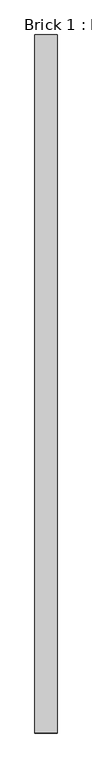
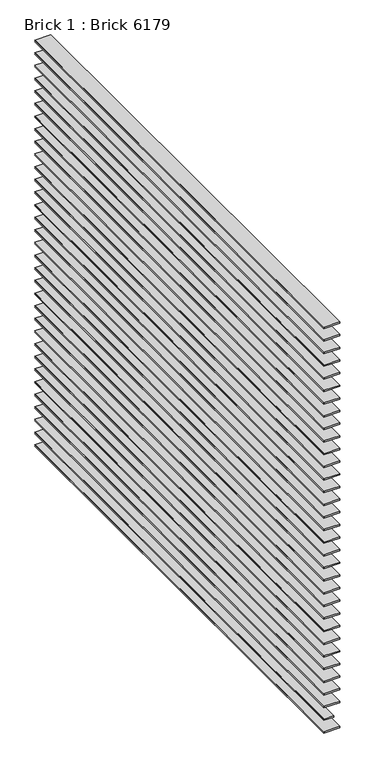
"""IFC4 building model written with IfcOpenShell, lengths in millimetres: proxy geometry, Brick 1 : Brick 6179."""

import ifcopenshell
import ifcopenshell.guid

model = None  # the IFC model being written
_history = None  # IfcOwnerHistory: only IFC2X3 demands one
_inside = {}  # id of a spatial element -> (the spatial element, [elements in it])
_under = {}  # id of a project, library or spatial element -> (it, [spatial elements below it])
_declared = {}  # id of a project -> (the project, [libraries it declares])
_typed = {}  # id of a type object -> (the type object, [elements of that type])
_made_of = {}  # id of a material, layer set ... -> (it, [elements and type objects made of it])


def new_model(schema):
    """Start an empty IFC model of exactly this schema.

    Asked for "IFC4X3", IfcOpenShell would pick the latest addendum, in which some entities
    have other attributes; the version numbers below select the first issue.
    IFC2X3 requires an IfcOwnerHistory on every rooted entity: one is made here for all.
    """
    global model, _history
    if schema == "IFC4X3":
        model = ifcopenshell.file(schema_version=(4, 3, 0, 0))
    else:
        model = ifcopenshell.file(schema=schema)
    _inside.clear()
    _under.clear()
    _declared.clear()
    _typed.clear()
    _made_of.clear()
    _history = None
    if model.schema == "IFC2X3":
        org = make("IfcOrganization", Name="unknown")
        user = make(
            "IfcPersonAndOrganization",
            ThePerson=make("IfcPerson", FamilyName="unknown"),
            TheOrganization=org,
        )
        app = make(
            "IfcApplication",
            ApplicationDeveloper=org,
            Version="unknown",
            ApplicationFullName="unknown",
            ApplicationIdentifier="unknown",
        )
        _history = make(
            "IfcOwnerHistory",
            OwningUser=user,
            OwningApplication=app,
            ChangeAction="ADDED",
            CreationDate=0,
        )
    return model


def make(cls, **values):
    """One entity of the class cls with the attributes given. An attribute that is None is left unset."""
    return model.create_entity(
        cls, **{name: value for name, value in values.items() if value is not None}
    )


def rooted(cls, **values):
    """An entity with a GlobalId (a new one), such as an element, a storey or a relation."""
    return make(cls, GlobalId=ifcopenshell.guid.new(), OwnerHistory=_history, **values)


def si_unit(unit_type, name, prefix=None):
    """IfcSIUnit, for example si_unit("LENGTHUNIT", "METRE", prefix="MILLI")."""
    return make("IfcSIUnit", UnitType=unit_type, Prefix=prefix, Name=name)


def assignment(units):
    """IfcUnitAssignment: the units of a project."""
    return None if units is None else make("IfcUnitAssignment", Units=units)


def point(xyz):
    """IfcCartesianPoint."""
    return None if xyz is None else make("IfcCartesianPoint", Coordinates=xyz)


def direction(xyz):
    """IfcDirection."""
    return None if xyz is None else make("IfcDirection", DirectionRatios=xyz)


def frame(location, z_axis=None, x_axis=None):
    """IfcAxis2Placement3D, a coordinate frame: its origin and axes. An axis left out is left unset."""
    return make(
        "IfcAxis2Placement3D",
        Location=point(location),
        Axis=direction(z_axis),
        RefDirection=direction(x_axis),
    )


def frame_2d(location, x_axis=None):
    """IfcAxis2Placement2D, a coordinate frame in the plane: its origin and x axis."""
    return make(
        "IfcAxis2Placement2D", Location=point(location), RefDirection=direction(x_axis)
    )


def origin():
    """The frame at (0, 0, 0) with its axes left unset."""
    return frame((0.0, 0.0, 0.0))


def place(relative_to, where):
    """IfcLocalPlacement: puts the frame where relative to a parent placement (None: the world)."""
    return make(
        "IfcLocalPlacement", PlacementRelTo=relative_to, RelativePlacement=where
    )


def context(
    kind, dimensions, precision=None, world=None, true_north=None, identifier=None
):
    """IfcGeometricRepresentationContext, for example the 3D "Model" context."""
    return make(
        "IfcGeometricRepresentationContext",
        ContextIdentifier=identifier,
        ContextType=kind,
        CoordinateSpaceDimension=dimensions,
        Precision=precision,
        WorldCoordinateSystem=world,
        TrueNorth=true_north,
    )


def project(units=None, contexts=None):
    """IfcProject with its units and contexts."""
    return rooted(
        "IfcProject",
        Name="project",
        RepresentationContexts=contexts,
        UnitsInContext=assignment(units),
    )


def spatial(cls, under=None, at=None, **own):
    """A site, building, storey or space (cls), placed at a placement, below another one or the project."""
    s = rooted(cls, ObjectPlacement=at, **own)
    if under is not None:
        _under.setdefault(under.id(), (under, []))[1].append(s)
    return s


def polyline(points):
    """IfcPolyline through the points."""
    return make("IfcPolyline", Points=[point(p) for p in points])


def circle_curve(where, radius):
    """IfcCircle in the frame where."""
    return make("IfcCircle", Position=where, Radius=radius)


def trimmed(basis, trim1, trim2, sense, master):
    """IfcTrimmedCurve: the piece of a basis curve between two trims."""
    return make(
        "IfcTrimmedCurve",
        BasisCurve=basis,
        Trim1=trim1,
        Trim2=trim2,
        SenseAgreement=sense,
        MasterRepresentation=master,
    )


def segment(curve, same_sense, transition):
    """IfcCompositeCurveSegment."""
    return make(
        "IfcCompositeCurveSegment",
        Transition=transition,
        SameSense=same_sense,
        ParentCurve=curve,
    )


def composite_curve(segments, self_intersect=None):
    """IfcCompositeCurve: segments joined end to end."""
    return make("IfcCompositeCurve", Segments=segments, SelfIntersect=self_intersect)


def outline(outer, holes=None, kind="AREA"):
    """IfcArbitraryClosedProfileDef: a profile drawn as a closed curve; with holes, ...WithVoids."""
    if holes is None:
        return make("IfcArbitraryClosedProfileDef", ProfileType=kind, OuterCurve=outer)
    return make(
        "IfcArbitraryProfileDefWithVoids",
        ProfileType=kind,
        OuterCurve=outer,
        InnerCurves=holes,
    )


def extrude(swept, where, along, depth):
    """IfcExtrudedAreaSolid: the profile swept, set in the frame where, extruded along a direction by depth."""
    return make(
        "IfcExtrudedAreaSolid",
        SweptArea=swept,
        Position=where,
        ExtrudedDirection=direction(along),
        Depth=depth,
    )


def shape(context_of_items, identifier, shape_type, items):
    """IfcShapeRepresentation: the items that make up one representation, for example the "Body"."""
    return make(
        "IfcShapeRepresentation",
        ContextOfItems=context_of_items,
        RepresentationIdentifier=identifier,
        RepresentationType=shape_type,
        Items=items,
    )


def source(mapping_origin, context_of_items, identifier, shape_type, items):
    """IfcRepresentationMap: a shape defined once, which mapped items show again and again."""
    return make(
        "IfcRepresentationMap",
        MappingOrigin=mapping_origin,
        MappedRepresentation=shape(context_of_items, identifier, shape_type, items),
    )


def transform(
    local_origin,
    x_axis=None,
    y_axis=None,
    z_axis=None,
    scale=None,
    scale2=None,
    scale3=None,
    uniform=True,
):
    """IfcCartesianTransformationOperator3D, or its non-uniform kind. x_axis, y_axis, z_axis: its Axis1, 2, 3."""
    if uniform:
        return make(
            "IfcCartesianTransformationOperator3D",
            Axis1=direction(x_axis),
            Axis2=direction(y_axis),
            LocalOrigin=point(local_origin),
            Scale=scale,
            Axis3=direction(z_axis),
        )
    return make(
        "IfcCartesianTransformationOperator3DnonUniform",
        Axis1=direction(x_axis),
        Axis2=direction(y_axis),
        LocalOrigin=point(local_origin),
        Scale=scale,
        Axis3=direction(z_axis),
        Scale2=scale2,
        Scale3=scale3,
    )


def mapped(mapping_source, mapping_target):
    """IfcMappedItem: shows the shape of a source again, moved by a transform."""
    return make(
        "IfcMappedItem", MappingSource=mapping_source, MappingTarget=mapping_target
    )


def made_of(thing, what):
    """Note that an element or type object is made of a material, layer set ...; save() writes the relation."""
    if what is not None:
        _made_of.setdefault(what.id(), (what, []))[1].append(thing)
    return thing


def element(
    cls,
    number,
    at=None,
    inside=None,
    cuts=None,
    type_object=None,
    material=None,
    context=None,
    identifier="Body",
    shape_type=None,
    held_by="IfcProductDefinitionShape",
    body=None,
    shapes=None,
    **own,
):
    """One element of the class cls, such as IfcWall. Its Tag is "e" and its number.

    at: its placement. inside: the storey or other place that contains it. cuts: it is an
    opening in that element (IfcRelVoidsElement). A single representation is given by context,
    identifier, shape_type and body (its items); several are given by shapes. held_by: the class
    of the entity that holds the representations. save() writes the other relations.
    """
    e = rooted(cls, Tag="e%d" % number, ObjectPlacement=at, **own)
    if body is not None:
        shapes = [shape(context, identifier, shape_type, body)]
    if shapes is not None:
        e.Representation = make(held_by, Representations=shapes)
    if inside is not None:
        _inside.setdefault(inside.id(), (inside, []))[1].append(e)
    if cuts is not None:
        rooted(
            "IfcRelVoidsElement", RelatingBuildingElement=cuts, RelatedOpeningElement=e
        )
    if type_object is not None:
        _typed.setdefault(type_object.id(), (type_object, []))[1].append(e)
    return made_of(e, material)


def aggregate(whole, parts):
    """IfcRelAggregates: a whole, such as a stair, and the parts it consists of."""
    return rooted("IfcRelAggregates", RelatingObject=whole, RelatedObjects=parts)


def save(model, path):
    """Write the relations noted so far, then the file.

    IfcRelAggregates (storeys below a building ...), IfcRelContainedInSpatialStructure (elements
    in a storey), IfcRelDefinesByType, IfcRelAssociatesMaterial and IfcRelDeclares: one each for
    every whole, place, type object, material and project.
    """
    for whole, parts in _under.values():
        aggregate(whole, parts)
    for where, things in _inside.values():
        rooted(
            "IfcRelContainedInSpatialStructure",
            RelatedElements=things,
            RelatingStructure=where,
        )
    for kind, things in _typed.values():
        rooted("IfcRelDefinesByType", RelatedObjects=things, RelatingType=kind)
    for what, things in _made_of.values():
        rooted("IfcRelAssociatesMaterial", RelatedObjects=things, RelatingMaterial=what)
    for by, libraries in _declared.values():
        rooted("IfcRelDeclares", RelatingContext=by, RelatedDefinitions=libraries)
    model.write(path)


def brick_1_brick_6179_25ec3522(model_context):
    return source(origin(), model_context, "Body", "SweptSolid", [
        extrude(outline(composite_curve([segment(polyline([(37320.25, 10083.0612048), (37326.2029111, 10083.0612048), (37326.2029111, 10019.5612048)]), True, "CONTINUOUS"), segment(trimmed(circle_curve(frame_2d((37323.2264555, 10016.8521801)), 4.0246867), [point((37326.2029111, 10019.5612048))], [point((37320.25, 10019.5612048))], True, "CARTESIAN"), True, "CONTINUOUS"), segment(polyline([(37320.25, 10019.5612048), (37320.25, 10083.0612048)]), True, "CONTINUOUS")], self_intersect=False)), frame((0.0, 2217.3609988, 0.0), z_axis=(0.0, 1.0, 0.0), x_axis=(0.0, 0.0, 1.0)), (0.0, 0.0, 1.0), 2000.0),
        extrude(outline(composite_curve([segment(polyline([(37373.6875, 10059.8947267), (37379.6404111, 10059.8947267), (37379.6404111, 10019.5612048)]), True, "CONTINUOUS"), segment(trimmed(circle_curve(frame_2d((37376.6639555, 10016.8521801)), 4.0246867), [point((37379.6404111, 10019.5612048))], [point((37373.6875, 10019.5612048))], True, "CARTESIAN"), True, "CONTINUOUS"), segment(polyline([(37373.6875, 10019.5612048), (37373.6875, 10059.8947267)]), True, "CONTINUOUS")], self_intersect=False)), frame((0.0, 2217.3609988, 0.0), z_axis=(0.0, 1.0, 0.0), x_axis=(0.0, 0.0, 1.0)), (0.0, 0.0, 1.0), 2000.0),
        extrude(outline(composite_curve([segment(polyline([(37427.125, 10083.0612048), (37433.0779111, 10083.0612048), (37433.0779111, 10019.5612048)]), True, "CONTINUOUS"), segment(trimmed(circle_curve(frame_2d((37430.1014555, 10016.8521801)), 4.0246867), [point((37433.0779111, 10019.5612048))], [point((37427.125, 10019.5612048))], True, "CARTESIAN"), True, "CONTINUOUS"), segment(polyline([(37427.125, 10019.5612048), (37427.125, 10083.0612048)]), True, "CONTINUOUS")], self_intersect=False)), frame((0.0, 2217.3609988, 0.0), z_axis=(0.0, 1.0, 0.0), x_axis=(0.0, 0.0, 1.0)), (0.0, 0.0, 1.0), 2000.0),
        extrude(outline(composite_curve([segment(polyline([(37480.5625, 10083.0612048), (37486.5154111, 10083.0612048), (37486.5154111, 10019.5612048)]), True, "CONTINUOUS"), segment(trimmed(circle_curve(frame_2d((37483.5389555, 10016.8521801)), 4.0246867), [point((37486.5154111, 10019.5612048))], [point((37480.5625, 10019.5612048))], True, "CARTESIAN"), True, "CONTINUOUS"), segment(polyline([(37480.5625, 10019.5612048), (37480.5625, 10083.0612048)]), True, "CONTINUOUS")], self_intersect=False)), frame((0.0, 2217.3609988, 0.0), z_axis=(0.0, 1.0, 0.0), x_axis=(0.0, 0.0, 1.0)), (0.0, 0.0, 1.0), 2000.0),
        extrude(outline(composite_curve([segment(polyline([(37534.0, 10083.0612048), (37539.9529111, 10083.0612048), (37539.9529111, 10019.5612048)]), True, "CONTINUOUS"), segment(trimmed(circle_curve(frame_2d((37536.9764555, 10016.8521801)), 4.0246867), [point((37539.9529111, 10019.5612048))], [point((37534.0, 10019.5612048))], True, "CARTESIAN"), True, "CONTINUOUS"), segment(polyline([(37534.0, 10019.5612048), (37534.0, 10083.0612048)]), True, "CONTINUOUS")], self_intersect=False)), frame((0.0, 2217.3609988, 0.0), z_axis=(0.0, 1.0, 0.0), x_axis=(0.0, 0.0, 1.0)), (0.0, 0.0, 1.0), 2000.0),
        extrude(outline(composite_curve([segment(polyline([(37587.4375, 10083.0612048), (37593.3904111, 10083.0612048), (37593.3904111, 10019.5612048)]), True, "CONTINUOUS"), segment(trimmed(circle_curve(frame_2d((37590.4139555, 10016.8521801)), 4.0246867), [point((37593.3904111, 10019.5612048))], [point((37587.4375, 10019.5612048))], True, "CARTESIAN"), True, "CONTINUOUS"), segment(polyline([(37587.4375, 10019.5612048), (37587.4375, 10083.0612048)]), True, "CONTINUOUS")], self_intersect=False)), frame((0.0, 2217.3609988, 0.0), z_axis=(0.0, 1.0, 0.0), x_axis=(0.0, 0.0, 1.0)), (0.0, 0.0, 1.0), 2000.0),
        extrude(outline(composite_curve([segment(polyline([(37640.875, 10083.0612048), (37646.8279111, 10083.0612048), (37646.8279111, 10019.5612048)]), True, "CONTINUOUS"), segment(trimmed(circle_curve(frame_2d((37643.8514555, 10016.8521801)), 4.0246867), [point((37646.8279111, 10019.5612048))], [point((37640.875, 10019.5612048))], True, "CARTESIAN"), True, "CONTINUOUS"), segment(polyline([(37640.875, 10019.5612048), (37640.875, 10083.0612048)]), True, "CONTINUOUS")], self_intersect=False)), frame((0.0, 2217.3609988, 0.0), z_axis=(0.0, 1.0, 0.0), x_axis=(0.0, 0.0, 1.0)), (0.0, 0.0, 1.0), 2000.0),
        extrude(outline(composite_curve([segment(polyline([(37694.3125, 10083.0612048), (37700.2654111, 10083.0612048), (37700.2654111, 10019.5612048)]), True, "CONTINUOUS"), segment(trimmed(circle_curve(frame_2d((37697.2889555, 10016.8521801)), 4.0246867), [point((37700.2654111, 10019.5612048))], [point((37694.3125, 10019.5612048))], True, "CARTESIAN"), True, "CONTINUOUS"), segment(polyline([(37694.3125, 10019.5612048), (37694.3125, 10083.0612048)]), True, "CONTINUOUS")], self_intersect=False)), frame((0.0, 2217.3609988, 0.0), z_axis=(0.0, 1.0, 0.0), x_axis=(0.0, 0.0, 1.0)), (0.0, 0.0, 1.0), 2000.0),
        extrude(outline(composite_curve([segment(polyline([(37747.75, 10083.0612048), (37753.7029111, 10083.0612048), (37753.7029111, 10019.5612048)]), True, "CONTINUOUS"), segment(trimmed(circle_curve(frame_2d((37750.7264555, 10016.8521801)), 4.0246867), [point((37753.7029111, 10019.5612048))], [point((37747.75, 10019.5612048))], True, "CARTESIAN"), True, "CONTINUOUS"), segment(polyline([(37747.75, 10019.5612048), (37747.75, 10083.0612048)]), True, "CONTINUOUS")], self_intersect=False)), frame((0.0, 2217.3609988, 0.0), z_axis=(0.0, 1.0, 0.0), x_axis=(0.0, 0.0, 1.0)), (0.0, 0.0, 1.0), 2000.0),
        extrude(outline(composite_curve([segment(polyline([(37801.1875, 10083.0612048), (37807.1404111, 10083.0612048), (37807.1404111, 10019.5612048)]), True, "CONTINUOUS"), segment(trimmed(circle_curve(frame_2d((37804.1639555, 10016.8521801)), 4.0246867), [point((37807.1404111, 10019.5612048))], [point((37801.1875, 10019.5612048))], True, "CARTESIAN"), True, "CONTINUOUS"), segment(polyline([(37801.1875, 10019.5612048), (37801.1875, 10083.0612048)]), True, "CONTINUOUS")], self_intersect=False)), frame((0.0, 2217.3609988, 0.0), z_axis=(0.0, 1.0, 0.0), x_axis=(0.0, 0.0, 1.0)), (0.0, 0.0, 1.0), 2000.0),
        extrude(outline(composite_curve([segment(polyline([(37854.625, 10083.0612048), (37860.5779111, 10083.0612048), (37860.5779111, 10019.5612048)]), True, "CONTINUOUS"), segment(trimmed(circle_curve(frame_2d((37857.6014555, 10016.8521801)), 4.0246867), [point((37860.5779111, 10019.5612048))], [point((37854.625, 10019.5612048))], True, "CARTESIAN"), True, "CONTINUOUS"), segment(polyline([(37854.625, 10019.5612048), (37854.625, 10083.0612048)]), True, "CONTINUOUS")], self_intersect=False)), frame((0.0, 2217.3609988, 0.0), z_axis=(0.0, 1.0, 0.0), x_axis=(0.0, 0.0, 1.0)), (0.0, 0.0, 1.0), 2000.0),
        extrude(outline(composite_curve([segment(polyline([(37908.0625, 10083.0612048), (37914.0154111, 10083.0612048), (37914.0154111, 10019.5612048)]), True, "CONTINUOUS"), segment(trimmed(circle_curve(frame_2d((37911.0389555, 10016.8521801)), 4.0246867), [point((37914.0154111, 10019.5612048))], [point((37908.0625, 10019.5612048))], True, "CARTESIAN"), True, "CONTINUOUS"), segment(polyline([(37908.0625, 10019.5612048), (37908.0625, 10083.0612048)]), True, "CONTINUOUS")], self_intersect=False)), frame((0.0, 2217.3609988, 0.0), z_axis=(0.0, 1.0, 0.0), x_axis=(0.0, 0.0, 1.0)), (0.0, 0.0, 1.0), 2000.0),
        extrude(outline(composite_curve([segment(polyline([(37961.5, 10083.0612048), (37967.4529111, 10083.0612048), (37967.4529111, 10019.5612048)]), True, "CONTINUOUS"), segment(trimmed(circle_curve(frame_2d((37964.4764555, 10016.8521801)), 4.0246867), [point((37967.4529111, 10019.5612048))], [point((37961.5, 10019.5612048))], True, "CARTESIAN"), True, "CONTINUOUS"), segment(polyline([(37961.5, 10019.5612048), (37961.5, 10083.0612048)]), True, "CONTINUOUS")], self_intersect=False)), frame((0.0, 2217.3609988, 0.0), z_axis=(0.0, 1.0, 0.0), x_axis=(0.0, 0.0, 1.0)), (0.0, 0.0, 1.0), 2000.0),
        extrude(outline(composite_curve([segment(polyline([(38014.9375, 10083.0612048), (38020.8904111, 10083.0612048), (38020.8904111, 10019.5612048)]), True, "CONTINUOUS"), segment(trimmed(circle_curve(frame_2d((38017.9139555, 10016.8521801)), 4.0246867), [point((38020.8904111, 10019.5612048))], [point((38014.9375, 10019.5612048))], True, "CARTESIAN"), True, "CONTINUOUS"), segment(polyline([(38014.9375, 10019.5612048), (38014.9375, 10083.0612048)]), True, "CONTINUOUS")], self_intersect=False)), frame((0.0, 2217.3609988, 0.0), z_axis=(0.0, 1.0, 0.0), x_axis=(0.0, 0.0, 1.0)), (0.0, 0.0, 1.0), 2000.0),
        extrude(outline(composite_curve([segment(polyline([(38068.375, 10083.0612048), (38074.3279111, 10083.0612048), (38074.3279111, 10019.5612048)]), True, "CONTINUOUS"), segment(trimmed(circle_curve(frame_2d((38071.3514555, 10016.8521801)), 4.0246867), [point((38074.3279111, 10019.5612048))], [point((38068.375, 10019.5612048))], True, "CARTESIAN"), True, "CONTINUOUS"), segment(polyline([(38068.375, 10019.5612048), (38068.375, 10083.0612048)]), True, "CONTINUOUS")], self_intersect=False)), frame((0.0, 2217.3609988, 0.0), z_axis=(0.0, 1.0, 0.0), x_axis=(0.0, 0.0, 1.0)), (0.0, 0.0, 1.0), 2000.0),
        extrude(outline(composite_curve([segment(polyline([(38121.8125, 10083.0612048), (38127.7654111, 10083.0612048), (38127.7654111, 10019.5612048)]), True, "CONTINUOUS"), segment(trimmed(circle_curve(frame_2d((38124.7889555, 10016.8521801)), 4.0246867), [point((38127.7654111, 10019.5612048))], [point((38121.8125, 10019.5612048))], True, "CARTESIAN"), True, "CONTINUOUS"), segment(polyline([(38121.8125, 10019.5612048), (38121.8125, 10083.0612048)]), True, "CONTINUOUS")], self_intersect=False)), frame((0.0, 2217.3609988, 0.0), z_axis=(0.0, 1.0, 0.0), x_axis=(0.0, 0.0, 1.0)), (0.0, 0.0, 1.0), 2000.0),
        extrude(outline(composite_curve([segment(polyline([(38175.25, 10083.0612048), (38181.2029111, 10083.0612048), (38181.2029111, 10019.5612048)]), True, "CONTINUOUS"), segment(trimmed(circle_curve(frame_2d((38178.2264555, 10016.8521801)), 4.0246867), [point((38181.2029111, 10019.5612048))], [point((38175.25, 10019.5612048))], True, "CARTESIAN"), True, "CONTINUOUS"), segment(polyline([(38175.25, 10019.5612048), (38175.25, 10083.0612048)]), True, "CONTINUOUS")], self_intersect=False)), frame((0.0, 2217.3609988, 0.0), z_axis=(0.0, 1.0, 0.0), x_axis=(0.0, 0.0, 1.0)), (0.0, 0.0, 1.0), 2000.0),
        extrude(outline(composite_curve([segment(polyline([(38228.6875, 10083.0612048), (38234.6404111, 10083.0612048), (38234.6404111, 10019.5612048)]), True, "CONTINUOUS"), segment(trimmed(circle_curve(frame_2d((38231.6639555, 10016.8521801)), 4.0246867), [point((38234.6404111, 10019.5612048))], [point((38228.6875, 10019.5612048))], True, "CARTESIAN"), True, "CONTINUOUS"), segment(polyline([(38228.6875, 10019.5612048), (38228.6875, 10083.0612048)]), True, "CONTINUOUS")], self_intersect=False)), frame((0.0, 2217.3609988, 0.0), z_axis=(0.0, 1.0, 0.0), x_axis=(0.0, 0.0, 1.0)), (0.0, 0.0, 1.0), 2000.0),
        extrude(outline(composite_curve([segment(polyline([(38282.125, 10083.0612048), (38288.0779111, 10083.0612048), (38288.0779111, 10019.5612048)]), True, "CONTINUOUS"), segment(trimmed(circle_curve(frame_2d((38285.1014555, 10016.8521801)), 4.0246867), [point((38288.0779111, 10019.5612048))], [point((38282.125, 10019.5612048))], True, "CARTESIAN"), True, "CONTINUOUS"), segment(polyline([(38282.125, 10019.5612048), (38282.125, 10083.0612048)]), True, "CONTINUOUS")], self_intersect=False)), frame((0.0, 2217.3609988, 0.0), z_axis=(0.0, 1.0, 0.0), x_axis=(0.0, 0.0, 1.0)), (0.0, 0.0, 1.0), 2000.0),
        extrude(outline(composite_curve([segment(polyline([(38335.5625, 10083.0612048), (38341.5154111, 10083.0612048), (38341.5154111, 10019.5612048)]), True, "CONTINUOUS"), segment(trimmed(circle_curve(frame_2d((38338.5389555, 10016.8521801)), 4.0246867), [point((38341.5154111, 10019.5612048))], [point((38335.5625, 10019.5612048))], True, "CARTESIAN"), True, "CONTINUOUS"), segment(polyline([(38335.5625, 10019.5612048), (38335.5625, 10083.0612048)]), True, "CONTINUOUS")], self_intersect=False)), frame((0.0, 2217.3609988, 0.0), z_axis=(0.0, 1.0, 0.0), x_axis=(0.0, 0.0, 1.0)), (0.0, 0.0, 1.0), 2000.0),
        extrude(outline(composite_curve([segment(polyline([(38389.0, 10083.0612048), (38394.9529111, 10083.0612048), (38394.9529111, 10019.5612048)]), True, "CONTINUOUS"), segment(trimmed(circle_curve(frame_2d((38391.9764555, 10016.8521801)), 4.0246867), [point((38394.9529111, 10019.5612048))], [point((38389.0, 10019.5612048))], True, "CARTESIAN"), True, "CONTINUOUS"), segment(polyline([(38389.0, 10019.5612048), (38389.0, 10083.0612048)]), True, "CONTINUOUS")], self_intersect=False)), frame((0.0, 2217.3609988, 0.0), z_axis=(0.0, 1.0, 0.0), x_axis=(0.0, 0.0, 1.0)), (0.0, 0.0, 1.0), 2000.0),
        extrude(outline(composite_curve([segment(polyline([(38442.4375, 10083.0612048), (38448.3904111, 10083.0612048), (38448.3904111, 10019.5612048)]), True, "CONTINUOUS"), segment(trimmed(circle_curve(frame_2d((38445.4139555, 10016.8521801)), 4.0246867), [point((38448.3904111, 10019.5612048))], [point((38442.4375, 10019.5612048))], True, "CARTESIAN"), True, "CONTINUOUS"), segment(polyline([(38442.4375, 10019.5612048), (38442.4375, 10083.0612048)]), True, "CONTINUOUS")], self_intersect=False)), frame((0.0, 2217.3609988, 0.0), z_axis=(0.0, 1.0, 0.0), x_axis=(0.0, 0.0, 1.0)), (0.0, 0.0, 1.0), 2000.0),
        extrude(outline(composite_curve([segment(polyline([(38495.875, 10083.0612048), (38501.8279111, 10083.0612048), (38501.8279111, 10019.5612048)]), True, "CONTINUOUS"), segment(trimmed(circle_curve(frame_2d((38498.8514555, 10016.8521801)), 4.0246867), [point((38501.8279111, 10019.5612048))], [point((38495.875, 10019.5612048))], True, "CARTESIAN"), True, "CONTINUOUS"), segment(polyline([(38495.875, 10019.5612048), (38495.875, 10083.0612048)]), True, "CONTINUOUS")], self_intersect=False)), frame((0.0, 2217.3609988, 0.0), z_axis=(0.0, 1.0, 0.0), x_axis=(0.0, 0.0, 1.0)), (0.0, 0.0, 1.0), 2000.0),
        extrude(outline(composite_curve([segment(polyline([(38549.3125, 10083.0612048), (38555.2654111, 10083.0612048), (38555.2654111, 10019.5612048)]), True, "CONTINUOUS"), segment(trimmed(circle_curve(frame_2d((38552.2889555, 10016.8521801)), 4.0246867), [point((38555.2654111, 10019.5612048))], [point((38549.3125, 10019.5612048))], True, "CARTESIAN"), True, "CONTINUOUS"), segment(polyline([(38549.3125, 10019.5612048), (38549.3125, 10083.0612048)]), True, "CONTINUOUS")], self_intersect=False)), frame((0.0, 2217.3609988, 0.0), z_axis=(0.0, 1.0, 0.0), x_axis=(0.0, 0.0, 1.0)), (0.0, 0.0, 1.0), 2000.0),
        extrude(outline(composite_curve([segment(polyline([(38602.75, 10083.0612048), (38608.7029111, 10083.0612048), (38608.7029111, 10019.5612048)]), True, "CONTINUOUS"), segment(trimmed(circle_curve(frame_2d((38605.7264555, 10016.8521801)), 4.0246867), [point((38608.7029111, 10019.5612048))], [point((38602.75, 10019.5612048))], True, "CARTESIAN"), True, "CONTINUOUS"), segment(polyline([(38602.75, 10019.5612048), (38602.75, 10083.0612048)]), True, "CONTINUOUS")], self_intersect=False)), frame((0.0, 2217.3609988, 0.0), z_axis=(0.0, 1.0, 0.0), x_axis=(0.0, 0.0, 1.0)), (0.0, 0.0, 1.0), 2000.0),
        extrude(outline(composite_curve([segment(polyline([(38656.1875, 10083.0612048), (38662.1404111, 10083.0612048), (38662.1404111, 10019.5612048)]), True, "CONTINUOUS"), segment(trimmed(circle_curve(frame_2d((38659.1639555, 10016.8521801)), 4.0246867), [point((38662.1404111, 10019.5612048))], [point((38656.1875, 10019.5612048))], True, "CARTESIAN"), True, "CONTINUOUS"), segment(polyline([(38656.1875, 10019.5612048), (38656.1875, 10083.0612048)]), True, "CONTINUOUS")], self_intersect=False)), frame((0.0, 2217.3609988, 0.0), z_axis=(0.0, 1.0, 0.0), x_axis=(0.0, 0.0, 1.0)), (0.0, 0.0, 1.0), 2000.0),
        extrude(outline(composite_curve([segment(polyline([(38709.625, 10083.0612048), (38715.5779111, 10083.0612048), (38715.5779111, 10019.5612048)]), True, "CONTINUOUS"), segment(trimmed(circle_curve(frame_2d((38712.6014555, 10016.8521801)), 4.0246867), [point((38715.5779111, 10019.5612048))], [point((38709.625, 10019.5612048))], True, "CARTESIAN"), True, "CONTINUOUS"), segment(polyline([(38709.625, 10019.5612048), (38709.625, 10083.0612048)]), True, "CONTINUOUS")], self_intersect=False)), frame((0.0, 2217.3609988, 0.0), z_axis=(0.0, 1.0, 0.0), x_axis=(0.0, 0.0, 1.0)), (0.0, 0.0, 1.0), 2000.0),
        extrude(outline(composite_curve([segment(polyline([(38763.0625, 10083.0612048), (38769.0154111, 10083.0612048), (38769.0154111, 10019.5612048)]), True, "CONTINUOUS"), segment(trimmed(circle_curve(frame_2d((38766.0389555, 10016.8521801)), 4.0246867), [point((38769.0154111, 10019.5612048))], [point((38763.0625, 10019.5612048))], True, "CARTESIAN"), True, "CONTINUOUS"), segment(polyline([(38763.0625, 10019.5612048), (38763.0625, 10083.0612048)]), True, "CONTINUOUS")], self_intersect=False)), frame((0.0, 2217.3609988, 0.0), z_axis=(0.0, 1.0, 0.0), x_axis=(0.0, 0.0, 1.0)), (0.0, 0.0, 1.0), 2000.0),
        extrude(outline(composite_curve([segment(polyline([(38816.5, 10083.0612048), (38822.4529111, 10083.0612048), (38822.4529111, 10019.5612048)]), True, "CONTINUOUS"), segment(trimmed(circle_curve(frame_2d((38819.4764555, 10016.8521801)), 4.0246867), [point((38822.4529111, 10019.5612048))], [point((38816.5, 10019.5612048))], True, "CARTESIAN"), True, "CONTINUOUS"), segment(polyline([(38816.5, 10019.5612048), (38816.5, 10083.0612048)]), True, "CONTINUOUS")], self_intersect=False)), frame((0.0, 2217.3609988, 0.0), z_axis=(0.0, 1.0, 0.0), x_axis=(0.0, 0.0, 1.0)), (0.0, 0.0, 1.0), 2000.0),
        extrude(outline(composite_curve([segment(polyline([(38869.9375, 10083.0612048), (38875.8904111, 10083.0612048), (38875.8904111, 10019.5612048)]), True, "CONTINUOUS"), segment(trimmed(circle_curve(frame_2d((38872.9139555, 10016.8521801)), 4.0246867), [point((38875.8904111, 10019.5612048))], [point((38869.9375, 10019.5612048))], True, "CARTESIAN"), True, "CONTINUOUS"), segment(polyline([(38869.9375, 10019.5612048), (38869.9375, 10083.0612048)]), True, "CONTINUOUS")], self_intersect=False)), frame((0.0, 2217.3609988, 0.0), z_axis=(0.0, 1.0, 0.0), x_axis=(0.0, 0.0, 1.0)), (0.0, 0.0, 1.0), 2000.0),
        extrude(outline(composite_curve([segment(polyline([(38923.375, 10083.0612048), (38929.3279111, 10083.0612048), (38929.3279111, 10019.5612048)]), True, "CONTINUOUS"), segment(trimmed(circle_curve(frame_2d((38926.3514555, 10016.8521801)), 4.0246867), [point((38929.3279111, 10019.5612048))], [point((38923.375, 10019.5612048))], True, "CARTESIAN"), True, "CONTINUOUS"), segment(polyline([(38923.375, 10019.5612048), (38923.375, 10083.0612048)]), True, "CONTINUOUS")], self_intersect=False)), frame((0.0, 2217.3609988, 0.0), z_axis=(0.0, 1.0, 0.0), x_axis=(0.0, 0.0, 1.0)), (0.0, 0.0, 1.0), 2000.0),
        extrude(outline(composite_curve([segment(polyline([(38976.8125, 10083.0612048), (38982.7654111, 10083.0612048), (38982.7654111, 10019.5612048)]), True, "CONTINUOUS"), segment(trimmed(circle_curve(frame_2d((38979.7889555, 10016.8521801)), 4.0246867), [point((38982.7654111, 10019.5612048))], [point((38976.8125, 10019.5612048))], True, "CARTESIAN"), True, "CONTINUOUS"), segment(polyline([(38976.8125, 10019.5612048), (38976.8125, 10083.0612048)]), True, "CONTINUOUS")], self_intersect=False)), frame((0.0, 2217.3609988, 0.0), z_axis=(0.0, 1.0, 0.0), x_axis=(0.0, 0.0, 1.0)), (0.0, 0.0, 1.0), 2000.0),
        extrude(outline(composite_curve([segment(polyline([(39030.25, 10083.0612048), (39036.2029111, 10083.0612048), (39036.2029111, 10019.5612048)]), True, "CONTINUOUS"), segment(trimmed(circle_curve(frame_2d((39033.2264555, 10016.8521801)), 4.0246867), [point((39036.2029111, 10019.5612048))], [point((39030.25, 10019.5612048))], True, "CARTESIAN"), True, "CONTINUOUS"), segment(polyline([(39030.25, 10019.5612048), (39030.25, 10083.0612048)]), True, "CONTINUOUS")], self_intersect=False)), frame((0.0, 2217.3609988, 0.0), z_axis=(0.0, 1.0, 0.0), x_axis=(0.0, 0.0, 1.0)), (0.0, 0.0, 1.0), 2000.0),
    ])


if __name__ == "__main__":
    model = new_model("IFC4")
    model_context = context("Model", 3, world=origin())
    ifc_project = project(units=[si_unit("LENGTHUNIT", "METRE", prefix="MILLI")], contexts=[model_context])
    site = spatial("IfcSite", under=ifc_project)
    building = spatial("IfcBuilding", under=site)
    placement = place(None, origin())
    brick_1_brick_6179_shape = brick_1_brick_6179_25ec3522(model_context)
    element("IfcBuildingElementProxy", 1, Name="Brick 1 : Brick 6179", ObjectType="Brick 1 : Brick 6179", at=placement, inside=building, context=model_context, shape_type="MappedRepresentation", body=[
        mapped(brick_1_brick_6179_shape, transform((0.0, 0.0, 0.0), x_axis=(1.0, 0.0, 0.0), y_axis=(0.0, 1.0, 0.0), z_axis=(0.0, 0.0, 1.0))),
    ])
    save(model, "model.ifc")

# Revit data of these elements
# Project information
#   Issued Date 1 = "0/00/2018 - City of Newport Beach"
#   IfcSite GUID = "3hCLsSIbaHwOLX093rt3ko"
#   IfcBuilding GUID = "3hCN2YIbaHwOLX093rt3ko"
#   IfcProject GUID = "7043067b_ee86_4e71_a94"
#   NameOverride = "Default Site"
#   Project Issue Date = "Issue Date"
#   Project Status = "Project Status"
#   Client Name = "xxx"
#   Project Address = "xxx"
#   Project Name = "STAUDENMEIER RESIDENCE"
# Type "Brick 1 : Brick 6179"
#   NameOverride = "Brick"
# Element 1 (IfcBuildingElementProxy, "Brick 1 : Brick 6179")
#   Materials on its faces: "MORTAR BED"
# Materials
#   "MORTAR BED": class "Unassigned", colour RGB 186 186 186, transparency 0, Cost = 0
